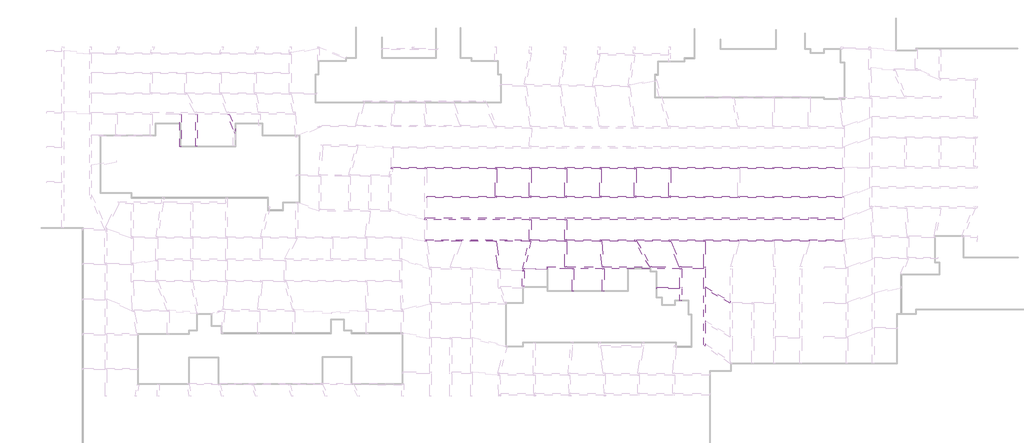
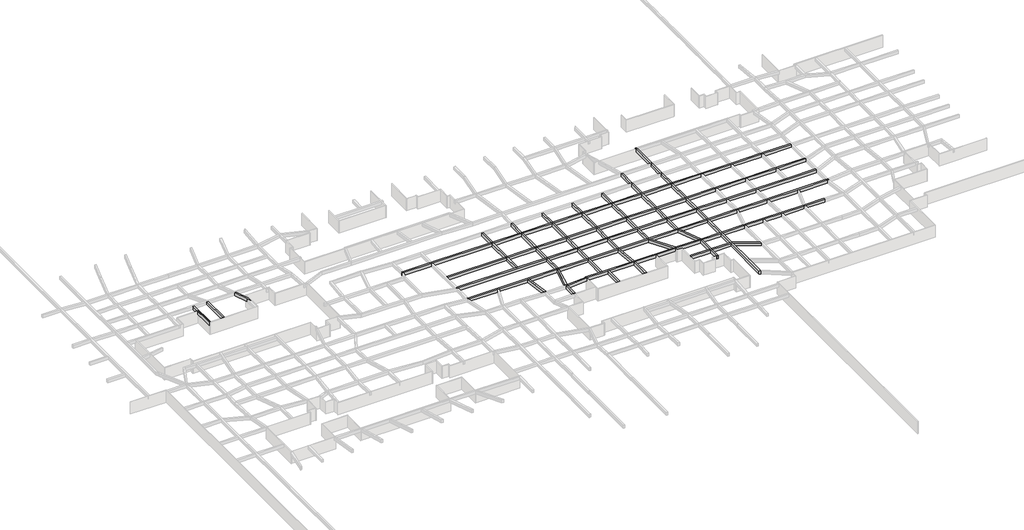
# One storey, part 18 of 45: 30 beams.
"""IFC4 building model written with IfcOpenShell, lengths in millimetres."""

from ifc_helpers import new_model, si_unit, frame, origin, place, context, project, spatial, polyline, outline, extrude, faceted_brep, element, save

model = new_model("IFC4")

# Units and contexts
model_context = context("Model", 3, world=origin())
ifc_project = project(units=[si_unit("LENGTHUNIT", "METRE", prefix="MILLI")], contexts=[model_context])

# Site, building, storey
site = spatial("IfcSite", under=ifc_project)
building = spatial("IfcBuilding", under=site)
storey = spatial("IfcBuildingStorey", under=building, Name="户型图", Elevation=0.0)

# Beams
placement = place(None, origin())
element("IfcBeam", 1, ObjectType="混凝土 - 矩形梁 : KL_beam", at=placement, inside=storey, context=model_context, shape_type="SweptSolid", body=[
    extrude(outline(polyline([(-119926.6222431, -61189.4871623), (-120326.6222431, -61189.4871623), (-120326.6222431, -53989.4871623), (-119926.6222431, -53989.4871623), (-119926.6222431, -61189.4871623)])), frame((0.0, 0.0, 2500.0), z_axis=(0.0, 0.0, 1.0), x_axis=(1.0, 0.0, 0.0)), (0.0, 0.0, 1.0), 800.0),
])
element("IfcBeam", 2, ObjectType="混凝土 - 矩形梁 : KL_beam", at=placement, inside=storey, context=model_context, shape_type="Brep", body=[
    faceted_brep([(-111449.0790859, -58416.1962178, 3300.0), (-111449.0790859, -57300.024974, 3300.0), (-112719.8754884, -53989.4871623, 3300.0), (-113148.3334859, -53989.4871623, 3300.0), (-111849.0790859, -57374.1605919, 3300.0), (-111449.0790859, -58416.1962178, 2500.0), (-113148.3334859, -53989.4871623, 2500.0), (-111849.0790859, -57374.1605919, 2500.0), (-111449.0790859, -57300.024974, 2500.0), (-112719.8754884, -53989.4871623, 2500.0)], [[[0, 1, 2, 3, 4]], [[5, 0, 4, 3, 6, 7]], [[8, 5, 7, 6, 9]], [[1, 8, 9, 2]], [[3, 2, 9, 6]], [[1, 0, 5, 8]]]),
])
element("IfcBeam", 3, ObjectType="混凝土 - 矩形梁 : KL_beam", at=placement, inside=storey, context=model_context, shape_type="SweptSolid", body=[
    extrude(outline(polyline([(-123526.6222431, -61289.4871623), (-123926.6222431, -61289.4871623), (-123926.6222431, -53989.4871623), (-123526.6222431, -53989.4871623), (-123526.6222431, -61289.4871623)])), frame((0.0, 0.0, 2500.0), z_axis=(0.0, 0.0, 1.0), x_axis=(1.0, 0.0, 0.0)), (0.0, 0.0, 1.0), 800.0),
])
element("IfcBeam", 4, ObjectType="混凝土 - 矩形梁 : KL_beam", at=placement, inside=storey, context=model_context, shape_type="Brep", body=[
    faceted_brep([(-76420.6999587, -65862.2662437, 3300.0), (-76420.6999587, -66034.5402932, 3300.0), (-76420.6999587, -66262.2662437, 3300.0), (-76069.4005138, -66262.2662437, 3300.0), (-68900.6999587, -66262.2662437, 3300.0), (-68500.6999587, -66262.2662437, 3300.0), (-53106.0296652, -66262.2662437, 3300.0), (-52706.0296652, -66262.2662437, 3300.0), (-45455.9166766, -66262.2662437, 3300.0), (-45055.9166766, -66262.2662437, 3300.0), (-37455.9166766, -66262.2662437, 3300.0), (-37055.9166766, -66262.2662437, 3300.0), (-29655.9166766, -66262.2662437, 3300.0), (-29255.9166766, -66262.2662437, 3300.0), (-21855.9166766, -66262.2662437, 3300.0), (-21455.9166766, -66262.2662437, 3300.0), (-14155.9166766, -66262.2662437, 3300.0), (-13755.9166766, -66262.2662437, 3300.0), (-6361.9880078, -66262.2662437, 3300.0), (-5961.9880078, -66262.2662437, 3300.0), (1338.0119922, -66262.2662437, 3300.0), (1738.0119922, -66262.2662437, 3300.0), (9138.0119922, -66262.2662437, 3300.0), (9538.0119922, -66262.2662437, 3300.0), (17160.5867178, -66262.2662437, 3300.0), (17560.5867178, -66262.2662437, 3300.0), (24866.4388689, -66262.2662437, 3300.0), (24866.4388689, -65862.2662437, 3300.0), (17560.5867178, -65862.2662437, 3300.0), (17160.5867178, -65862.2662437, 3300.0), (9538.0119922, -65862.2662437, 3300.0), (9138.0119922, -65862.2662437, 3300.0), (1738.0119922, -65862.2662437, 3300.0), (1338.0119922, -65862.2662437, 3300.0), (-5961.9880078, -65862.2662437, 3300.0), (-6361.9880078, -65862.2662437, 3300.0), (-13755.9166766, -65862.2662437, 3300.0), (-14155.9166766, -65862.2662437, 3300.0), (-21455.9166766, -65862.2662437, 3300.0), (-21855.9166766, -65862.2662437, 3300.0), (-29255.9166766, -65862.2662437, 3300.0), (-29655.9166766, -65862.2662437, 3300.0), (-37055.9166766, -65862.2662437, 3300.0), (-37455.9166766, -65862.2662437, 3300.0), (-45055.9166766, -65862.2662437, 3300.0), (-45455.9166766, -65862.2662437, 3300.0), (-52706.0296652, -65862.2662437, 3300.0), (-53106.0296652, -65862.2662437, 3300.0), (-68500.6999587, -65862.2662437, 3300.0), (-68900.6999587, -65862.2662437, 3300.0), (-76020.6999587, -65862.2662437, 3300.0), (-76420.6999587, -66262.2662437, 2500.0), (-76069.4005138, -66262.2662437, 2500.0), (-68900.6999587, -66262.2662437, 2500.0), (-68500.6999587, -66262.2662437, 2500.0), (-53106.0296652, -66262.2662437, 2500.0), (-52706.0296652, -66262.2662437, 2500.0), (-45455.9166766, -66262.2662437, 2500.0), (-45055.9166766, -66262.2662437, 2500.0), (-37455.9166766, -66262.2662437, 2500.0), (-37055.9166766, -66262.2662437, 2500.0), (-29655.9166766, -66262.2662437, 2500.0), (-29255.9166766, -66262.2662437, 2500.0), (-21855.9166766, -66262.2662437, 2500.0), (-21455.9166766, -66262.2662437, 2500.0), (-14155.9166766, -66262.2662437, 2500.0), (-13755.9166766, -66262.2662437, 2500.0), (-6361.9880078, -66262.2662437, 2500.0), (-5961.9880078, -66262.2662437, 2500.0), (1338.0119922, -66262.2662437, 2500.0), (1738.0119922, -66262.2662437, 2500.0), (9138.0119922, -66262.2662437, 2500.0), (9538.0119922, -66262.2662437, 2500.0), (17160.5867178, -66262.2662437, 2500.0), (17560.5867178, -66262.2662437, 2500.0), (24866.4388689, -66262.2662437, 2500.0), (-76420.6999587, -66034.5402932, 2500.0), (-76420.6999587, -65862.2662437, 2500.0), (-76020.6999587, -65862.2662437, 2500.0), (-68900.6999587, -65862.2662437, 2500.0), (-68500.6999587, -65862.2662437, 2500.0), (-53106.0296652, -65862.2662437, 2500.0), (-52706.0296652, -65862.2662437, 2500.0), (-45455.9166766, -65862.2662437, 2500.0), (-45055.9166766, -65862.2662437, 2500.0), (-37455.9166766, -65862.2662437, 2500.0), (-37055.9166766, -65862.2662437, 2500.0), (-29655.9166766, -65862.2662437, 2500.0), (-29255.9166766, -65862.2662437, 2500.0), (-21855.9166766, -65862.2662437, 2500.0), (-21455.9166766, -65862.2662437, 2500.0), (-14155.9166766, -65862.2662437, 2500.0), (-13755.9166766, -65862.2662437, 2500.0), (-6361.9880078, -65862.2662437, 2500.0), (-5961.9880078, -65862.2662437, 2500.0), (1338.0119922, -65862.2662437, 2500.0), (1738.0119922, -65862.2662437, 2500.0), (9138.0119922, -65862.2662437, 2500.0), (9538.0119922, -65862.2662437, 2500.0), (17160.5867178, -65862.2662437, 2500.0), (17560.5867178, -65862.2662437, 2500.0), (24866.4388689, -65862.2662437, 2500.0)], [[[0, 1, 2, 3, 4, 5, 6, 7, 8, 9, 10, 11, 12, 13, 14, 15, 16, 17, 18, 19, 20, 21, 22, 23, 24, 25, 26, 27, 28, 29, 30, 31, 32, 33, 34, 35, 36, 37, 38, 39, 40, 41, 42, 43, 44, 45, 46, 47, 48, 49, 50]], [[2, 51, 52, 53, 54, 55, 56, 57, 58, 59, 60, 61, 62, 63, 64, 65, 66, 67, 68, 69, 70, 71, 72, 73, 74, 75, 26, 25, 24, 23, 22, 21, 20, 19, 18, 17, 16, 15, 14, 13, 12, 11, 10, 9, 8, 7, 6, 5, 4, 3]], [[51, 76, 77, 78, 79, 80, 81, 82, 83, 84, 85, 86, 87, 88, 89, 90, 91, 92, 93, 94, 95, 96, 97, 98, 99, 100, 101, 75, 74, 73, 72, 71, 70, 69, 68, 67, 66, 65, 64, 63, 62, 61, 60, 59, 58, 57, 56, 55, 54, 53, 52]], [[77, 0, 50, 49, 48, 47, 46, 45, 44, 43, 42, 41, 40, 39, 38, 37, 36, 35, 34, 33, 32, 31, 30, 29, 28, 27, 101, 100, 99, 98, 97, 96, 95, 94, 93, 92, 91, 90, 89, 88, 87, 86, 85, 84, 83, 82, 81, 80, 79, 78]], [[2, 1, 0, 77, 76, 51]], [[27, 26, 75, 101]]]),
])
element("IfcBeam", 5, ObjectType="混凝土 - 矩形梁 : KL_beam", at=placement, inside=storey, context=model_context, shape_type="Brep", body=[
    faceted_brep([(-68500.6999587, -72411.6769994, 3300.0), (-68500.6999587, -72811.6769994, 3300.0), (-53106.0296652, -72811.6769994, 3300.0), (-52706.0296652, -72811.6769994, 3300.0), (-45455.9166766, -72811.6769994, 3300.0), (-45055.9166766, -72811.6769994, 3300.0), (-37455.9166766, -72811.6769994, 3300.0), (-37055.9166766, -72811.6769994, 3300.0), (-29655.9166766, -72811.6769994, 3300.0), (-29255.9166766, -72811.6769994, 3300.0), (-21855.9166766, -72811.6769994, 3300.0), (-21455.9166766, -72811.6769994, 3300.0), (-14155.9166766, -72811.6769994, 3300.0), (-13755.9166766, -72811.6769994, 3300.0), (-6361.9880078, -72811.6769994, 3300.0), (-5961.9880078, -72811.6769994, 3300.0), (1338.0119922, -72811.6769994, 3300.0), (1738.0119922, -72811.6769994, 3300.0), (9138.0119922, -72811.6769994, 3300.0), (9538.0119922, -72811.6769994, 3300.0), (17160.5867178, -72811.6769994, 3300.0), (17560.5867178, -72811.6769994, 3300.0), (24866.4388689, -72811.6769994, 3300.0), (24866.4388689, -72411.6769994, 3300.0), (17560.5867178, -72411.6769994, 3300.0), (17160.5867178, -72411.6769994, 3300.0), (9538.0119922, -72411.6769994, 3300.0), (9138.0119922, -72411.6769994, 3300.0), (1738.0119922, -72411.6769994, 3300.0), (1338.0119922, -72411.6769994, 3300.0), (-5961.9880078, -72411.6769994, 3300.0), (-6361.9880078, -72411.6769994, 3300.0), (-13755.9166766, -72411.6769994, 3300.0), (-14155.9166766, -72411.6769994, 3300.0), (-21455.9166766, -72411.6769994, 3300.0), (-21855.9166766, -72411.6769994, 3300.0), (-29255.9166766, -72411.6769994, 3300.0), (-29655.9166766, -72411.6769994, 3300.0), (-37055.9166766, -72411.6769994, 3300.0), (-37455.9166766, -72411.6769994, 3300.0), (-45055.9166766, -72411.6769994, 3300.0), (-45455.9166766, -72411.6769994, 3300.0), (-52706.0296652, -72411.6769994, 3300.0), (-53106.0296652, -72411.6769994, 3300.0), (-68500.6999587, -72811.6769994, 2500.0), (-53106.0296652, -72811.6769994, 2500.0), (-52706.0296652, -72811.6769994, 2500.0), (-45455.9166766, -72811.6769994, 2500.0), (-45055.9166766, -72811.6769994, 2500.0), (-37455.9166766, -72811.6769994, 2500.0), (-37055.9166766, -72811.6769994, 2500.0), (-29655.9166766, -72811.6769994, 2500.0), (-29255.9166766, -72811.6769994, 2500.0), (-21855.9166766, -72811.6769994, 2500.0), (-21455.9166766, -72811.6769994, 2500.0), (-14155.9166766, -72811.6769994, 2500.0), (-13755.9166766, -72811.6769994, 2500.0), (-6361.9880078, -72811.6769994, 2500.0), (-5961.9880078, -72811.6769994, 2500.0), (1338.0119922, -72811.6769994, 2500.0), (1738.0119922, -72811.6769994, 2500.0), (9138.0119922, -72811.6769994, 2500.0), (9538.0119922, -72811.6769994, 2500.0), (17160.5867178, -72811.6769994, 2500.0), (17560.5867178, -72811.6769994, 2500.0), (24866.4388689, -72811.6769994, 2500.0), (-68500.6999587, -72411.6769994, 2500.0), (-53106.0296652, -72411.6769994, 2500.0), (-52706.0296652, -72411.6769994, 2500.0), (-45455.9166766, -72411.6769994, 2500.0), (-45055.9166766, -72411.6769994, 2500.0), (-37455.9166766, -72411.6769994, 2500.0), (-37055.9166766, -72411.6769994, 2500.0), (-29655.9166766, -72411.6769994, 2500.0), (-29255.9166766, -72411.6769994, 2500.0), (-21855.9166766, -72411.6769994, 2500.0), (-21455.9166766, -72411.6769994, 2500.0), (-14155.9166766, -72411.6769994, 2500.0), (-13755.9166766, -72411.6769994, 2500.0), (-6361.9880078, -72411.6769994, 2500.0), (-5961.9880078, -72411.6769994, 2500.0), (1338.0119922, -72411.6769994, 2500.0), (1738.0119922, -72411.6769994, 2500.0), (9138.0119922, -72411.6769994, 2500.0), (9538.0119922, -72411.6769994, 2500.0), (17160.5867178, -72411.6769994, 2500.0), (17560.5867178, -72411.6769994, 2500.0), (24866.4388689, -72411.6769994, 2500.0)], [[[0, 1, 2, 3, 4, 5, 6, 7, 8, 9, 10, 11, 12, 13, 14, 15, 16, 17, 18, 19, 20, 21, 22, 23, 24, 25, 26, 27, 28, 29, 30, 31, 32, 33, 34, 35, 36, 37, 38, 39, 40, 41, 42, 43]], [[1, 44, 45, 46, 47, 48, 49, 50, 51, 52, 53, 54, 55, 56, 57, 58, 59, 60, 61, 62, 63, 64, 65, 22, 21, 20, 19, 18, 17, 16, 15, 14, 13, 12, 11, 10, 9, 8, 7, 6, 5, 4, 3, 2]], [[44, 66, 67, 68, 69, 70, 71, 72, 73, 74, 75, 76, 77, 78, 79, 80, 81, 82, 83, 84, 85, 86, 87, 65, 64, 63, 62, 61, 60, 59, 58, 57, 56, 55, 54, 53, 52, 51, 50, 49, 48, 47, 46, 45]], [[66, 0, 43, 42, 41, 40, 39, 38, 37, 36, 35, 34, 33, 32, 31, 30, 29, 28, 27, 26, 25, 24, 23, 87, 86, 85, 84, 83, 82, 81, 80, 79, 78, 77, 76, 75, 74, 73, 72, 71, 70, 69, 68, 67]], [[1, 0, 66, 44]], [[23, 22, 65, 87]]]),
])
element("IfcBeam", 6, ObjectType="混凝土 - 矩形梁 : KL_beam", at=placement, inside=storey, context=model_context, shape_type="Brep", body=[
    faceted_brep([(-68900.6999587, -77289.9052253, 3300.0), (-68900.6999587, -77321.0496242, 3300.0), (-68900.6999587, -77689.9052253, 3300.0), (-68500.6999587, -77689.9052253, 3300.0), (-45455.9166766, -77689.9052253, 3300.0), (-45055.9166766, -77689.9052253, 3300.0), (-37455.9166766, -77689.9052253, 3300.0), (-37055.9166766, -77689.9052253, 3300.0), (-29655.9166766, -77689.9052253, 3300.0), (-29255.9166766, -77689.9052253, 3300.0), (-21855.9166766, -77689.9052253, 3300.0), (-21455.9166766, -77689.9052253, 3300.0), (-14155.9166766, -77689.9052253, 3300.0), (-13755.9166766, -77689.9052253, 3300.0), (-6361.9880078, -77689.9052253, 3300.0), (-5961.9880078, -77689.9052253, 3300.0), (1338.0119922, -77689.9052253, 3300.0), (1738.0119922, -77689.9052253, 3300.0), (9138.0119922, -77689.9052253, 3300.0), (9538.0119922, -77689.9052253, 3300.0), (24866.4388689, -77689.9052253, 3300.0), (24866.4388689, -77289.9052253, 3300.0), (17560.5867178, -77289.9052253, 3300.0), (17160.5867178, -77289.9052253, 3300.0), (9538.0119922, -77289.9052253, 3300.0), (9138.0119922, -77289.9052253, 3300.0), (1738.0119922, -77289.9052253, 3300.0), (1338.0119922, -77289.9052253, 3300.0), (-5961.9880078, -77289.9052253, 3300.0), (-6361.9880078, -77289.9052253, 3300.0), (-13755.9166766, -77289.9052253, 3300.0), (-14155.9166766, -77289.9052253, 3300.0), (-21455.9166766, -77289.9052253, 3300.0), (-21855.9166766, -77289.9052253, 3300.0), (-29255.9166766, -77289.9052253, 3300.0), (-29655.9166766, -77289.9052253, 3300.0), (-37055.9166766, -77289.9052253, 3300.0), (-37455.9166766, -77289.9052253, 3300.0), (-45055.9166766, -77289.9052253, 3300.0), (-45455.9166766, -77289.9052253, 3300.0), (-52706.0296652, -77289.9052253, 3300.0), (-53106.0296652, -77289.9052253, 3300.0), (-68500.6999587, -77289.9052253, 3300.0), (-68900.6999587, -77689.9052253, 2500.0), (-68500.6999587, -77689.9052253, 2500.0), (-45455.9166766, -77689.9052253, 2500.0), (-45055.9166766, -77689.9052253, 2500.0), (-37455.9166766, -77689.9052253, 2500.0), (-37055.9166766, -77689.9052253, 2500.0), (-29655.9166766, -77689.9052253, 2500.0), (-29255.9166766, -77689.9052253, 2500.0), (-21855.9166766, -77689.9052253, 2500.0), (-21455.9166766, -77689.9052253, 2500.0), (-14155.9166766, -77689.9052253, 2500.0), (-13755.9166766, -77689.9052253, 2500.0), (-6361.9880078, -77689.9052253, 2500.0), (-5961.9880078, -77689.9052253, 2500.0), (1338.0119922, -77689.9052253, 2500.0), (1738.0119922, -77689.9052253, 2500.0), (9138.0119922, -77689.9052253, 2500.0), (9538.0119922, -77689.9052253, 2500.0), (24866.4388689, -77689.9052253, 2500.0), (-68900.6999587, -77321.0496242, 2500.0), (-68900.6999587, -77289.9052253, 2500.0), (-68500.6999587, -77289.9052253, 2500.0), (-53106.0296652, -77289.9052253, 2500.0), (-52706.0296652, -77289.9052253, 2500.0), (-45455.9166766, -77289.9052253, 2500.0), (-45055.9166766, -77289.9052253, 2500.0), (-37455.9166766, -77289.9052253, 2500.0), (-37055.9166766, -77289.9052253, 2500.0), (-29655.9166766, -77289.9052253, 2500.0), (-29255.9166766, -77289.9052253, 2500.0), (-21855.9166766, -77289.9052253, 2500.0), (-21455.9166766, -77289.9052253, 2500.0), (-14155.9166766, -77289.9052253, 2500.0), (-13755.9166766, -77289.9052253, 2500.0), (-6361.9880078, -77289.9052253, 2500.0), (-5961.9880078, -77289.9052253, 2500.0), (1338.0119922, -77289.9052253, 2500.0), (1738.0119922, -77289.9052253, 2500.0), (9138.0119922, -77289.9052253, 2500.0), (9538.0119922, -77289.9052253, 2500.0), (17160.5867178, -77289.9052253, 2500.0), (17560.5867178, -77289.9052253, 2500.0), (24866.4388689, -77289.9052253, 2500.0)], [[[0, 1, 2, 3, 4, 5, 6, 7, 8, 9, 10, 11, 12, 13, 14, 15, 16, 17, 18, 19, 20, 21, 22, 23, 24, 25, 26, 27, 28, 29, 30, 31, 32, 33, 34, 35, 36, 37, 38, 39, 40, 41, 42]], [[2, 43, 44, 45, 46, 47, 48, 49, 50, 51, 52, 53, 54, 55, 56, 57, 58, 59, 60, 61, 20, 19, 18, 17, 16, 15, 14, 13, 12, 11, 10, 9, 8, 7, 6, 5, 4, 3]], [[43, 62, 63, 64, 65, 66, 67, 68, 69, 70, 71, 72, 73, 74, 75, 76, 77, 78, 79, 80, 81, 82, 83, 84, 85, 61, 60, 59, 58, 57, 56, 55, 54, 53, 52, 51, 50, 49, 48, 47, 46, 45, 44]], [[63, 0, 42, 41, 40, 39, 38, 37, 36, 35, 34, 33, 32, 31, 30, 29, 28, 27, 26, 25, 24, 23, 22, 21, 85, 84, 83, 82, 81, 80, 79, 78, 77, 76, 75, 74, 73, 72, 71, 70, 69, 68, 67, 66, 65, 64]], [[2, 1, 0, 63, 62, 43]], [[21, 20, 61, 85]]]),
])
element("IfcBeam", 7, ObjectType="混凝土 - 矩形梁 : KL_beam", at=placement, inside=storey, context=model_context, shape_type="Brep", body=[
    faceted_brep([(-68721.961123, -82134.4617231, 3300.0), (-68745.1611393, -82534.4617231, 3300.0), (-68495.5196461, -82534.4617231, 3300.0), (-61086.3295601, -82534.4617231, 3300.0), (-60660.6584511, -82534.4617231, 3300.0), (-53214.7333467, -82534.4617231, 3300.0), (-52811.3449172, -82534.4617231, 3300.0), (-45507.3511364, -82534.4617231, 3300.0), (-45096.8294933, -82534.4617231, 3300.0), (-37455.9166766, -82534.4617231, 3300.0), (-37055.9166766, -82534.4617231, 3300.0), (-29638.00353, -82534.4617231, 3300.0), (-29236.2432002, -82534.4617231, 3300.0), (-21771.3867304, -82534.4617231, 3300.0), (-21309.5065151, -82534.4617231, 3300.0), (-14090.81838, -82534.4617231, 3300.0), (-13659.4044829, -82534.4617231, 3300.0), (-6361.9880078, -82534.4617231, 3300.0), (-5961.9880078, -82534.4617231, 3300.0), (1277.3669177, -82534.4617231, 3300.0), (1691.4773898, -82534.4617231, 3300.0), (9144.8742373, -82534.4617231, 3300.0), (9545.118055, -82534.4617231, 3300.0), (17090.3022302, -82534.4617231, 3300.0), (17508.5789328, -82534.4617231, 3300.0), (24889.5407453, -82534.4617231, 3300.0), (25266.4388689, -82534.4617231, 3300.0), (25266.4388689, -82511.406776, 3300.0), (25266.4388689, -82134.4617231, 3300.0), (24866.4388689, -82134.4617231, 3300.0), (9538.0119922, -82134.4617231, 3300.0), (9138.0119922, -82134.4617231, 3300.0), (1738.0119922, -82134.4617231, 3300.0), (1338.0119922, -82134.4617231, 3300.0), (-5961.9880078, -82134.4617231, 3300.0), (-6361.9880078, -82134.4617231, 3300.0), (-13755.9166766, -82134.4617231, 3300.0), (-14155.9166766, -82134.4617231, 3300.0), (-21455.9166766, -82134.4617231, 3300.0), (-21855.9166766, -82134.4617231, 3300.0), (-29255.9166766, -82134.4617231, 3300.0), (-29655.9166766, -82134.4617231, 3300.0), (-37055.9166766, -82134.4617231, 3300.0), (-37455.9166766, -82134.4617231, 3300.0), (-45055.9166766, -82134.4617231, 3300.0), (-45455.9166766, -82134.4617231, 3300.0), (-68500.6999587, -82134.4617231, 3300.0), (-68745.1611393, -82534.4617231, 2500.0), (-68495.5196461, -82534.4617231, 2500.0), (-61086.3295601, -82534.4617231, 2500.0), (-60660.6584511, -82534.4617231, 2500.0), (-53214.7333467, -82534.4617231, 2500.0), (-52811.3449172, -82534.4617231, 2500.0), (-45507.3511364, -82534.4617231, 2500.0), (-45096.8294933, -82534.4617231, 2500.0), (-37455.9166766, -82534.4617231, 2500.0), (-37055.9166766, -82534.4617231, 2500.0), (-29638.00353, -82534.4617231, 2500.0), (-29236.2432002, -82534.4617231, 2500.0), (-21771.3867304, -82534.4617231, 2500.0), (-21309.5065151, -82534.4617231, 2500.0), (-14090.81838, -82534.4617231, 2500.0), (-13659.4044829, -82534.4617231, 2500.0), (-6361.9880078, -82534.4617231, 2500.0), (-5961.9880078, -82534.4617231, 2500.0), (1277.3669177, -82534.4617231, 2500.0), (1691.4773898, -82534.4617231, 2500.0), (9144.8742373, -82534.4617231, 2500.0), (9545.118055, -82534.4617231, 2500.0), (17090.3022302, -82534.4617231, 2500.0), (17508.5789328, -82534.4617231, 2500.0), (24889.5407453, -82534.4617231, 2500.0), (25266.4388689, -82534.4617231, 2500.0), (-68721.961123, -82134.4617231, 2500.0), (-68500.6999587, -82134.4617231, 2500.0), (-45455.9166766, -82134.4617231, 2500.0), (-45055.9166766, -82134.4617231, 2500.0), (-37455.9166766, -82134.4617231, 2500.0), (-37055.9166766, -82134.4617231, 2500.0), (-29655.9166766, -82134.4617231, 2500.0), (-29255.9166766, -82134.4617231, 2500.0), (-21855.9166766, -82134.4617231, 2500.0), (-21455.9166766, -82134.4617231, 2500.0), (-14155.9166766, -82134.4617231, 2500.0), (-13755.9166766, -82134.4617231, 2500.0), (-6361.9880078, -82134.4617231, 2500.0), (-5961.9880078, -82134.4617231, 2500.0), (1338.0119922, -82134.4617231, 2500.0), (1738.0119922, -82134.4617231, 2500.0), (9138.0119922, -82134.4617231, 2500.0), (9538.0119922, -82134.4617231, 2500.0), (24866.4388689, -82134.4617231, 2500.0), (25266.4388689, -82134.4617231, 2500.0), (25266.4388689, -82511.406776, 2500.0)], [[[0, 1, 2, 3, 4, 5, 6, 7, 8, 9, 10, 11, 12, 13, 14, 15, 16, 17, 18, 19, 20, 21, 22, 23, 24, 25, 26, 27, 28, 29, 30, 31, 32, 33, 34, 35, 36, 37, 38, 39, 40, 41, 42, 43, 44, 45, 46]], [[1, 47, 48, 49, 50, 51, 52, 53, 54, 55, 56, 57, 58, 59, 60, 61, 62, 63, 64, 65, 66, 67, 68, 69, 70, 71, 72, 26, 25, 24, 23, 22, 21, 20, 19, 18, 17, 16, 15, 14, 13, 12, 11, 10, 9, 8, 7, 6, 5, 4, 3, 2]], [[47, 73, 74, 75, 76, 77, 78, 79, 80, 81, 82, 83, 84, 85, 86, 87, 88, 89, 90, 91, 92, 93, 72, 71, 70, 69, 68, 67, 66, 65, 64, 63, 62, 61, 60, 59, 58, 57, 56, 55, 54, 53, 52, 51, 50, 49, 48]], [[73, 0, 46, 45, 44, 43, 42, 41, 40, 39, 38, 37, 36, 35, 34, 33, 32, 31, 30, 29, 28, 92, 91, 90, 89, 88, 87, 86, 85, 84, 83, 82, 81, 80, 79, 78, 77, 76, 75, 74]], [[0, 73, 47, 1]], [[28, 27, 26, 72, 93, 92]]]),
])
element("IfcBeam", 8, ObjectType="混凝土 - 矩形梁 : KL_beam", at=placement, inside=storey, context=model_context, shape_type="Brep", body=[
    faceted_brep([(-41470.268972, -88390.7983183, 3300.0), (-41451.2732989, -88687.9389906, 3300.0), (-41444.7497786, -88789.9834517, 3300.0), (-41444.7497786, -88789.9834517, 2500.0), (-41451.2732989, -88687.9389906, 2500.0), (-41470.268972, -88390.7983183, 2500.0), (-41477.971202, -88391.2907081, 3300.0), (-46523.4512037, -88713.8392437, 3300.0), (-46785.1341431, -88730.5681671, 3300.0), (-46772.3615365, -89130.5681671, 3300.0), (-46578.6472042, -89118.1843555, 3300.0), (-46772.3615365, -89130.5681671, 2500.0), (-46578.6472042, -89118.1843555, 2500.0), (-46785.1341431, -88730.5681671, 2500.0), (-46523.4512037, -88713.8392437, 2500.0), (-41477.971202, -88391.2907081, 2500.0)], [[[0, 1, 2, 3, 4, 5]], [[2, 1, 0, 6, 7, 8, 9, 10]], [[3, 2, 10, 9, 11, 12]], [[5, 4, 3, 12, 11, 13, 14, 15]], [[0, 5, 15, 14, 13, 8, 7, 6]], [[8, 13, 11, 9]]]),
])
element("IfcBeam", 9, ObjectType="混凝土 - 矩形梁 : KL_beam", at=placement, inside=storey, context=model_context, shape_type="SweptSolid", body=[
    extrude(outline(polyline([(-52173.5106555, -88730.5681671), (-52408.1333935, -88718.2721105), (-53214.7333467, -82534.4617231), (-52811.3449172, -82534.4617231), (-52003.1410987, -88730.5681671), (-52173.5106555, -88730.5681671)])), frame((0.0, 0.0, 2500.0), z_axis=(0.0, 0.0, 1.0), x_axis=(1.0, 0.0, 0.0)), (0.0, 0.0, 1.0), 800.0),
])
element("IfcBeam", 10, ObjectType="混凝土 - 矩形梁 : KL_beam", at=placement, inside=storey, context=model_context, shape_type="SweptSolid", body=[
    extrude(outline(polyline([(-46578.6472042, -92630.5681671), (-46978.6472042, -92630.5681671), (-46978.6472042, -89130.5681671), (-46772.3615365, -89130.5681671), (-46578.6472042, -89118.1843555), (-46578.6472042, -92630.5681671)])), frame((0.0, 0.0, 2500.0), z_axis=(0.0, 0.0, 1.0), x_axis=(1.0, 0.0, 0.0)), (0.0, 0.0, 1.0), 800.0),
])
element("IfcBeam", 11, ObjectType="混凝土 - 矩形梁 : KL_beam", at=placement, inside=storey, context=model_context, shape_type="SweptSolid", body=[
    extrude(outline(polyline([(-46785.1341431, -88730.5681671), (-46937.8350231, -88730.5681671), (-45507.3511364, -82534.4617231), (-45096.8294933, -82534.4617231), (-46523.4512037, -88713.8392437), (-46785.1341431, -88730.5681671)])), frame((0.0, 0.0, 2500.0), z_axis=(0.0, 0.0, 1.0), x_axis=(1.0, 0.0, 0.0)), (0.0, 0.0, 1.0), 800.0),
])
element("IfcBeam", 12, ObjectType="混凝土 - 矩形梁 : KL_beam", at=placement, inside=storey, context=model_context, shape_type="SweptSolid", body=[
    extrude(outline(polyline([(-45455.9166766, -77689.9052253), (-45055.9166766, -77689.9052253), (-45055.9166766, -82134.4617231), (-45455.9166766, -82134.4617231), (-45455.9166766, -77689.9052253)])), frame((0.0, 0.0, 2500.0), z_axis=(0.0, 0.0, 1.0), x_axis=(1.0, 0.0, 0.0)), (0.0, 0.0, 1.0), 800.0),
])
element("IfcBeam", 13, ObjectType="混凝土 - 矩形梁 : KL_beam", at=placement, inside=storey, context=model_context, shape_type="SweptSolid", body=[
    extrude(outline(polyline([(-37455.9166766, -77689.9052253), (-37055.9166766, -77689.9052253), (-37055.9166766, -82134.4617231), (-37455.9166766, -82134.4617231), (-37455.9166766, -77689.9052253)])), frame((0.0, 0.0, 2500.0), z_axis=(0.0, 0.0, 1.0), x_axis=(1.0, 0.0, 0.0)), (0.0, 0.0, 1.0), 800.0),
])
element("IfcBeam", 14, ObjectType="混凝土 - 矩形梁 : KL_beam", at=placement, inside=storey, context=model_context, shape_type="SweptSolid", body=[
    extrude(outline(polyline([(-53106.0296652, -61644.2645659), (-52706.0296652, -61644.2645659), (-52706.0296652, -65862.2662437), (-53106.0296652, -65862.2662437), (-53106.0296652, -61644.2645659)])), frame((0.0, 0.0, 2500.0), z_axis=(0.0, 0.0, 1.0), x_axis=(1.0, 0.0, 0.0)), (0.0, 0.0, 1.0), 800.0),
    extrude(outline(polyline([(-52706.0296652, -77289.9052253), (-53106.0296652, -77289.9052253), (-53106.0296652, -72811.6769994), (-52706.0296652, -72811.6769994), (-52706.0296652, -77289.9052253)])), frame((0.0, 0.0, 2500.0), z_axis=(0.0, 0.0, 1.0), x_axis=(1.0, 0.0, 0.0)), (0.0, 0.0, 1.0), 800.0),
    extrude(outline(polyline([(-53106.0296652, -66262.2662437), (-52706.0296652, -66262.2662437), (-52706.0296652, -72411.6769994), (-53106.0296652, -72411.6769994), (-53106.0296652, -66262.2662437)])), frame((0.0, 0.0, 2500.0), z_axis=(0.0, 0.0, 1.0), x_axis=(1.0, 0.0, 0.0)), (0.0, 0.0, 1.0), 800.0),
])
element("IfcBeam", 15, ObjectType="混凝土 - 矩形梁 : KL_beam", at=placement, inside=storey, context=model_context, shape_type="SweptSolid", body=[
    extrude(outline(polyline([(-45455.9166766, -61644.2645659), (-45055.9166766, -61644.2645659), (-45055.9166766, -65862.2662437), (-45455.9166766, -65862.2662437), (-45455.9166766, -61644.2645659)])), frame((0.0, 0.0, 2500.0), z_axis=(0.0, 0.0, 1.0), x_axis=(1.0, 0.0, 0.0)), (0.0, 0.0, 1.0), 800.0),
    extrude(outline(polyline([(-45055.9166766, -77289.9052253), (-45455.9166766, -77289.9052253), (-45455.9166766, -72811.6769994), (-45055.9166766, -72811.6769994), (-45055.9166766, -77289.9052253)])), frame((0.0, 0.0, 2500.0), z_axis=(0.0, 0.0, 1.0), x_axis=(1.0, 0.0, 0.0)), (0.0, 0.0, 1.0), 800.0),
    extrude(outline(polyline([(-45455.9166766, -66262.2662437), (-45055.9166766, -66262.2662437), (-45055.9166766, -72411.6769994), (-45455.9166766, -72411.6769994), (-45455.9166766, -66262.2662437)])), frame((0.0, 0.0, 2500.0), z_axis=(0.0, 0.0, 1.0), x_axis=(1.0, 0.0, 0.0)), (0.0, 0.0, 1.0), 800.0),
])
element("IfcBeam", 16, ObjectType="混凝土 - 矩形梁 : KL_beam", at=placement, inside=storey, context=model_context, shape_type="SweptSolid", body=[
    extrude(outline(polyline([(-37455.9166766, -61644.2645659), (-37055.9166766, -61644.2645659), (-37055.9166766, -65862.2662437), (-37455.9166766, -65862.2662437), (-37455.9166766, -61644.2645659)])), frame((0.0, 0.0, 2500.0), z_axis=(0.0, 0.0, 1.0), x_axis=(1.0, 0.0, 0.0)), (0.0, 0.0, 1.0), 800.0),
    extrude(outline(polyline([(-37055.9166766, -77289.9052253), (-37455.9166766, -77289.9052253), (-37455.9166766, -72811.6769994), (-37055.9166766, -72811.6769994), (-37055.9166766, -77289.9052253)])), frame((0.0, 0.0, 2500.0), z_axis=(0.0, 0.0, 1.0), x_axis=(1.0, 0.0, 0.0)), (0.0, 0.0, 1.0), 800.0),
    extrude(outline(polyline([(-37455.9166766, -66262.2662437), (-37055.9166766, -66262.2662437), (-37055.9166766, -72411.6769994), (-37455.9166766, -72411.6769994), (-37455.9166766, -66262.2662437)])), frame((0.0, 0.0, 2500.0), z_axis=(0.0, 0.0, 1.0), x_axis=(1.0, 0.0, 0.0)), (0.0, 0.0, 1.0), 800.0),
])
element("IfcBeam", 17, ObjectType="混凝土 - 矩形梁 : KL_beam", at=placement, inside=storey, context=model_context, shape_type="SweptSolid", body=[
    extrude(outline(polyline([(-29655.9166766, -61644.2645659), (-29255.9166766, -61644.2645659), (-29255.9166766, -65862.2662437), (-29655.9166766, -65862.2662437), (-29655.9166766, -61644.2645659)])), frame((0.0, 0.0, 2500.0), z_axis=(0.0, 0.0, 1.0), x_axis=(1.0, 0.0, 0.0)), (0.0, 0.0, 1.0), 800.0),
    extrude(outline(polyline([(-29255.9166766, -82134.4617231), (-29655.9166766, -82134.4617231), (-29655.9166766, -77689.9052253), (-29255.9166766, -77689.9052253), (-29255.9166766, -82134.4617231)])), frame((0.0, 0.0, 2500.0), z_axis=(0.0, 0.0, 1.0), x_axis=(1.0, 0.0, 0.0)), (0.0, 0.0, 1.0), 800.0),
    extrude(outline(polyline([(-29655.9166766, -66262.2662437), (-29255.9166766, -66262.2662437), (-29255.9166766, -72411.6769994), (-29655.9166766, -72411.6769994), (-29655.9166766, -66262.2662437)])), frame((0.0, 0.0, 2500.0), z_axis=(0.0, 0.0, 1.0), x_axis=(1.0, 0.0, 0.0)), (0.0, 0.0, 1.0), 800.0),
    extrude(outline(polyline([(-29655.9166766, -72811.6769994), (-29255.9166766, -72811.6769994), (-29255.9166766, -77289.9052253), (-29655.9166766, -77289.9052253), (-29655.9166766, -72811.6769994)])), frame((0.0, 0.0, 2500.0), z_axis=(0.0, 0.0, 1.0), x_axis=(1.0, 0.0, 0.0)), (0.0, 0.0, 1.0), 800.0),
])
element("IfcBeam", 18, ObjectType="混凝土 - 矩形梁 : KL_beam", at=placement, inside=storey, context=model_context, shape_type="SweptSolid", body=[
    extrude(outline(polyline([(-21855.9166766, -61644.2645659), (-21455.9166766, -61644.2645659), (-21455.9166766, -65862.2662437), (-21855.9166766, -65862.2662437), (-21855.9166766, -61644.2645659)])), frame((0.0, 0.0, 2500.0), z_axis=(0.0, 0.0, 1.0), x_axis=(1.0, 0.0, 0.0)), (0.0, 0.0, 1.0), 800.0),
    extrude(outline(polyline([(-21455.9166766, -82134.4617231), (-21855.9166766, -82134.4617231), (-21855.9166766, -77689.9052253), (-21455.9166766, -77689.9052253), (-21455.9166766, -82134.4617231)])), frame((0.0, 0.0, 2500.0), z_axis=(0.0, 0.0, 1.0), x_axis=(1.0, 0.0, 0.0)), (0.0, 0.0, 1.0), 800.0),
    extrude(outline(polyline([(-21855.9166766, -66262.2662437), (-21455.9166766, -66262.2662437), (-21455.9166766, -72411.6769994), (-21855.9166766, -72411.6769994), (-21855.9166766, -66262.2662437)])), frame((0.0, 0.0, 2500.0), z_axis=(0.0, 0.0, 1.0), x_axis=(1.0, 0.0, 0.0)), (0.0, 0.0, 1.0), 800.0),
    extrude(outline(polyline([(-21855.9166766, -72811.6769994), (-21455.9166766, -72811.6769994), (-21455.9166766, -77289.9052253), (-21855.9166766, -77289.9052253), (-21855.9166766, -72811.6769994)])), frame((0.0, 0.0, 2500.0), z_axis=(0.0, 0.0, 1.0), x_axis=(1.0, 0.0, 0.0)), (0.0, 0.0, 1.0), 800.0),
])
element("IfcBeam", 19, ObjectType="混凝土 - 矩形梁 : KL_beam", at=placement, inside=storey, context=model_context, shape_type="SweptSolid", body=[
    extrude(outline(polyline([(-13755.9166766, -82134.4617231), (-14155.9166766, -82134.4617231), (-14155.9166766, -77689.9052253), (-13755.9166766, -77689.9052253), (-13755.9166766, -82134.4617231)])), frame((0.0, 0.0, 2500.0), z_axis=(0.0, 0.0, 1.0), x_axis=(1.0, 0.0, 0.0)), (0.0, 0.0, 1.0), 800.0),
    extrude(outline(polyline([(-14155.9166766, -57112.697306), (-13755.9166766, -57112.697306), (-13755.9166766, -61244.2645659), (-14155.9166766, -61244.2645659), (-14155.9166766, -57112.697306)])), frame((0.0, 0.0, 2500.0), z_axis=(0.0, 0.0, 1.0), x_axis=(1.0, 0.0, 0.0)), (0.0, 0.0, 1.0), 800.0),
    extrude(outline(polyline([(-14155.9166766, -61644.2645659), (-13755.9166766, -61644.2645659), (-13755.9166766, -65862.2662437), (-14155.9166766, -65862.2662437), (-14155.9166766, -61644.2645659)])), frame((0.0, 0.0, 2500.0), z_axis=(0.0, 0.0, 1.0), x_axis=(1.0, 0.0, 0.0)), (0.0, 0.0, 1.0), 800.0),
    extrude(outline(polyline([(-14155.9166766, -66262.2662437), (-13755.9166766, -66262.2662437), (-13755.9166766, -72411.6769994), (-14155.9166766, -72411.6769994), (-14155.9166766, -66262.2662437)])), frame((0.0, 0.0, 2500.0), z_axis=(0.0, 0.0, 1.0), x_axis=(1.0, 0.0, 0.0)), (0.0, 0.0, 1.0), 800.0),
    extrude(outline(polyline([(-14155.9166766, -72811.6769994), (-13755.9166766, -72811.6769994), (-13755.9166766, -77289.9052253), (-14155.9166766, -77289.9052253), (-14155.9166766, -72811.6769994)])), frame((0.0, 0.0, 2500.0), z_axis=(0.0, 0.0, 1.0), x_axis=(1.0, 0.0, 0.0)), (0.0, 0.0, 1.0), 800.0),
])
element("IfcBeam", 20, ObjectType="混凝土 - 矩形梁 : KL_beam", at=placement, inside=storey, context=model_context, shape_type="Brep", body=[
    faceted_brep([(-6361.9880078, -105772.1367475, 3300.0), (-5961.9880078, -106053.71057, 3300.0), (-5961.9880078, -105564.5441182, 3300.0), (-5961.9880078, -100834.7253412, 3300.0), (-5961.9880078, -100372.6431355, 3300.0), (-5961.9880078, -93214.7253412, 3300.0), (-5961.9880078, -92752.6431355, 3300.0), (-5961.9880078, -88687.9389906, 3300.0), (-5961.9880078, -88287.9389906, 3300.0), (-5961.9880078, -82534.4617231, 3300.0), (-6361.9880078, -82534.4617231, 3300.0), (-6361.9880078, -88287.9389906, 3300.0), (-6361.9880078, -88687.9389906, 3300.0), (-6361.9880078, -92793.9793842, 3300.0), (-6361.9880078, -93193.9793842, 3300.0), (-6361.9880078, -105772.1367475, 2500.0), (-6361.9880078, -82534.4617231, 2500.0), (-6361.9880078, -88287.9389906, 2500.0), (-6361.9880078, -88687.9389906, 2500.0), (-6361.9880078, -92793.9793842, 2500.0), (-6361.9880078, -93193.9793842, 2500.0), (-5961.9880078, -106053.71057, 2500.0), (-5961.9880078, -82534.4617231, 2500.0), (-5961.9880078, -88287.9389906, 2500.0), (-5961.9880078, -88687.9389906, 2500.0), (-5961.9880078, -92752.6431355, 2500.0), (-5961.9880078, -93214.7253412, 2500.0), (-5961.9880078, -100372.6431355, 2500.0), (-5961.9880078, -100834.7253412, 2500.0), (-5961.9880078, -105564.5441182, 2500.0)], [[[0, 1, 2, 3, 4, 5, 6, 7, 8, 9, 10, 11, 12, 13, 14]], [[15, 0, 14, 13, 12, 11, 10, 16, 17, 18, 19, 20]], [[21, 15, 20, 19, 18, 17, 16, 22, 23, 24, 25, 26, 27, 28, 29]], [[1, 21, 29, 28, 27, 26, 25, 24, 23, 22, 9, 8, 7, 6, 5, 4, 3, 2]], [[10, 9, 22, 16]], [[1, 0, 15, 21]]]),
    faceted_brep([(-6361.9880078, -57112.697306, 3300.0), (-5961.9880078, -57112.697306, 3300.0), (-5961.9880078, -57112.697306, 2500.0), (-6361.9880078, -57112.697306, 2500.0), (-5961.9880078, -61244.2645659, 3300.0), (-6361.9880078, -61244.2645659, 3300.0), (-6361.9880078, -61244.2645659, 2500.0), (-5961.9880078, -61244.2645659, 2500.0)], [[[0, 1, 2, 3]], [[4, 5, 6, 7]], [[1, 0, 5, 4]], [[0, 3, 6, 5]], [[3, 2, 7, 6]], [[2, 1, 4, 7]]]),
    faceted_brep([(-5961.9880078, -56712.697306, 3300.0), (-6361.9880078, -56712.697306, 3300.0), (-6361.9880078, -56712.697306, 2500.0), (-5961.9880078, -56712.697306, 2500.0), (-5961.9880078, -50434.4617231, 3300.0), (-5961.9880078, -50034.4617231, 3300.0), (-6361.9880078, -50034.4617231, 3300.0), (-6361.9880078, -50034.4617231, 2500.0), (-5961.9880078, -50034.4617231, 2500.0), (-5961.9880078, -50434.4617231, 2500.0)], [[[0, 1, 2, 3]], [[1, 0, 4, 5, 6]], [[2, 1, 6, 7]], [[3, 2, 7, 8, 9]], [[0, 3, 9, 8, 5, 4]], [[6, 5, 8, 7]]]),
    faceted_brep([(-6361.9880078, -61644.2645659, 3300.0), (-5961.9880078, -61644.2645659, 3300.0), (-5961.9880078, -61644.2645659, 2500.0), (-6361.9880078, -61644.2645659, 2500.0), (-5961.9880078, -65862.2662437, 3300.0), (-6361.9880078, -65862.2662437, 3300.0), (-6361.9880078, -65862.2662437, 2500.0), (-5961.9880078, -65862.2662437, 2500.0)], [[[0, 1, 2, 3]], [[4, 5, 6, 7]], [[1, 0, 5, 4]], [[0, 3, 6, 5]], [[3, 2, 7, 6]], [[2, 1, 4, 7]]]),
    faceted_brep([(-6361.9880078, -66262.2662437, 3300.0), (-5961.9880078, -66262.2662437, 3300.0), (-5961.9880078, -66262.2662437, 2500.0), (-6361.9880078, -66262.2662437, 2500.0), (-5961.9880078, -72411.6769994, 3300.0), (-6361.9880078, -72411.6769994, 3300.0), (-6361.9880078, -72411.6769994, 2500.0), (-5961.9880078, -72411.6769994, 2500.0)], [[[0, 1, 2, 3]], [[4, 5, 6, 7]], [[1, 0, 5, 4]], [[0, 3, 6, 5]], [[3, 2, 7, 6]], [[2, 1, 4, 7]]]),
    faceted_brep([(-6361.9880078, -72811.6769994, 3300.0), (-5961.9880078, -72811.6769994, 3300.0), (-5961.9880078, -72811.6769994, 2500.0), (-6361.9880078, -72811.6769994, 2500.0), (-5961.9880078, -77289.9052253, 3300.0), (-6361.9880078, -77289.9052253, 3300.0), (-6361.9880078, -77289.9052253, 2500.0), (-5961.9880078, -77289.9052253, 2500.0)], [[[0, 1, 2, 3]], [[4, 5, 6, 7]], [[1, 0, 5, 4]], [[0, 3, 6, 5]], [[3, 2, 7, 6]], [[2, 1, 4, 7]]]),
    faceted_brep([(-6361.9880078, -77689.9052253, 3300.0), (-5961.9880078, -77689.9052253, 3300.0), (-5961.9880078, -77689.9052253, 2500.0), (-6361.9880078, -77689.9052253, 2500.0), (-5961.9880078, -82134.4617231, 3300.0), (-6361.9880078, -82134.4617231, 3300.0), (-6361.9880078, -82134.4617231, 2500.0), (-5961.9880078, -82134.4617231, 2500.0)], [[[0, 1, 2, 3]], [[4, 5, 6, 7]], [[1, 0, 5, 4]], [[0, 3, 6, 5]], [[3, 2, 7, 6]], [[2, 1, 4, 7]]]),
])
element("IfcBeam", 21, ObjectType="混凝土 - 矩形梁 : KL_beam", at=placement, inside=storey, context=model_context, shape_type="Brep", body=[
    faceted_brep([(-41477.971202, -88287.9389906, 3300.0), (-41477.971202, -88287.9389906, 2500.0), (-41477.971202, -88391.2907081, 2500.0), (-41477.971202, -88391.2907081, 3300.0), (-41470.268972, -88390.7983183, 3300.0), (-41451.2732989, -88687.9389906, 3300.0), (-35863.8297061, -88687.9389906, 3300.0), (-35463.8297061, -88687.9389906, 3300.0), (-29077.9505198, -88687.9389906, 3300.0), (-28677.9505198, -88687.9389906, 3300.0), (-11669.7015983, -88687.9389906, 3300.0), (-11269.7015983, -88687.9389906, 3300.0), (-6361.9880078, -88687.9389906, 3300.0), (-6361.9880078, -88287.9389906, 3300.0), (-11334.8487771, -88287.9389906, 3300.0), (-11766.2626742, -88287.9389906, 3300.0), (-17987.7348659, -88287.9389906, 3300.0), (-18449.6150813, -88287.9389906, 3300.0), (-28695.8750901, -88287.9389906, 3300.0), (-29097.6354199, -88287.9389906, 3300.0), (-37055.9166766, -88287.9389906, 3300.0), (-37455.9166766, -88287.9389906, 3300.0), (-6361.9880078, -88287.9389906, 2500.0), (-11334.8487771, -88287.9389906, 2500.0), (-11766.2626742, -88287.9389906, 2500.0), (-17987.7348659, -88287.9389906, 2500.0), (-18449.6150813, -88287.9389906, 2500.0), (-28695.8750901, -88287.9389906, 2500.0), (-29097.6354199, -88287.9389906, 2500.0), (-37055.9166766, -88287.9389906, 2500.0), (-37455.9166766, -88287.9389906, 2500.0), (-6361.9880078, -88687.9389906, 2500.0), (-11269.7015983, -88687.9389906, 2500.0), (-11669.7015983, -88687.9389906, 2500.0), (-28677.9505198, -88687.9389906, 2500.0), (-29077.9505198, -88687.9389906, 2500.0), (-35463.8297061, -88687.9389906, 2500.0), (-35863.8297061, -88687.9389906, 2500.0), (-41451.2732989, -88687.9389906, 2500.0), (-41470.268972, -88390.7983183, 2500.0)], [[[0, 1, 2, 3]], [[0, 3, 4, 5, 6, 7, 8, 9, 10, 11, 12, 13, 14, 15, 16, 17, 18, 19, 20, 21]], [[1, 0, 21, 20, 19, 18, 17, 16, 15, 14, 13, 22, 23, 24, 25, 26, 27, 28, 29, 30]], [[2, 1, 30, 29, 28, 27, 26, 25, 24, 23, 22, 31, 32, 33, 34, 35, 36, 37, 38, 39]], [[5, 38, 37, 36, 35, 34, 33, 32, 31, 12, 11, 10, 9, 8, 7, 6]], [[4, 39, 38, 5]], [[39, 4, 3, 2]], [[13, 12, 31, 22]]]),
    faceted_brep([(20722.028798, -88687.9389906, 3300.0), (20722.028798, -88687.9389906, 2500.0), (20722.028798, -88287.9389906, 2500.0), (20722.028798, -88287.9389906, 3300.0), (-5961.9880078, -88687.9389906, 3300.0), (-5961.9880078, -88287.9389906, 3300.0), (-5961.9880078, -88287.9389906, 2500.0), (-5961.9880078, -88687.9389906, 2500.0), (15749.5644071, -88287.9389906, 3300.0), (15331.2877045, -88287.9389906, 3300.0), (9746.0339084, -88287.9389906, 3300.0), (9345.7900907, -88287.9389906, 3300.0), (149.8378023, -88287.9389906, 3300.0), (-264.2726698, -88287.9389906, 3300.0), (-310.8072722, -88687.9389906, 3300.0), (89.1927278, -88687.9389906, 3300.0), (4489.1927278, -88687.9389906, 3300.0), (4889.1927278, -88687.9389906, 3300.0), (9352.8961535, -88687.9389906, 3300.0), (9752.8961535, -88687.9389906, 3300.0), (15279.3735446, -88687.9389906, 3300.0), (15679.3735446, -88687.9389906, 3300.0), (15749.5644071, -88287.9389906, 2500.0), (15331.2877045, -88287.9389906, 2500.0), (9746.0339084, -88287.9389906, 2500.0), (9345.7900907, -88287.9389906, 2500.0), (149.8378023, -88287.9389906, 2500.0), (-264.2726698, -88287.9389906, 2500.0), (15679.3735446, -88687.9389906, 2500.0), (15279.3735446, -88687.9389906, 2500.0), (9752.8961535, -88687.9389906, 2500.0), (9352.8961535, -88687.9389906, 2500.0), (4889.1927278, -88687.9389906, 2500.0), (4489.1927278, -88687.9389906, 2500.0), (89.1927278, -88687.9389906, 2500.0), (-310.8072722, -88687.9389906, 2500.0)], [[[0, 1, 2, 3]], [[4, 5, 6, 7]], [[0, 3, 8, 9, 10, 11, 12, 13, 5, 4, 14, 15, 16, 17, 18, 19, 20, 21]], [[3, 2, 22, 23, 24, 25, 26, 27, 6, 5, 13, 12, 11, 10, 9, 8]], [[2, 1, 28, 29, 30, 31, 32, 33, 34, 35, 7, 6, 27, 26, 25, 24, 23, 22]], [[1, 0, 21, 20, 19, 18, 17, 16, 15, 14, 4, 7, 35, 34, 33, 32, 31, 30, 29, 28]]]),
])
element("IfcBeam", 22, ObjectType="混凝土 - 矩形梁 : KL_beam", at=placement, inside=storey, context=model_context, shape_type="SweptSolid", body=[
    extrude(outline(polyline([(-29638.00353, -82534.4617231), (-29236.2432002, -82534.4617231), (-28695.8750901, -88287.9389906), (-29097.6354199, -88287.9389906), (-29638.00353, -82534.4617231)])), frame((0.0, 0.0, 2500.0), z_axis=(0.0, 0.0, 1.0), x_axis=(1.0, 0.0, 0.0)), (0.0, 0.0, 1.0), 800.0),
])
element("IfcBeam", 23, ObjectType="混凝土 - 矩形梁 : KL_beam", at=placement, inside=storey, context=model_context, shape_type="SweptSolid", body=[
    extrude(outline(polyline([(-21771.3867304, -82534.4617231), (-21309.5065151, -82534.4617231), (-17987.7348659, -88287.9389906), (-18449.6150813, -88287.9389906), (-21771.3867304, -82534.4617231)])), frame((0.0, 0.0, 2500.0), z_axis=(0.0, 0.0, 1.0), x_axis=(1.0, 0.0, 0.0)), (0.0, 0.0, 1.0), 800.0),
])
element("IfcBeam", 24, ObjectType="混凝土 - 矩形梁 : KL_beam", at=placement, inside=storey, context=model_context, shape_type="SweptSolid", body=[
    extrude(outline(polyline([(-14090.81838, -82534.4617231), (-13659.4044829, -82534.4617231), (-11334.8487771, -88287.9389906), (-11766.2626742, -88287.9389906), (-14090.81838, -82534.4617231)])), frame((0.0, 0.0, 2500.0), z_axis=(0.0, 0.0, 1.0), x_axis=(1.0, 0.0, 0.0)), (0.0, 0.0, 1.0), 800.0),
])
element("IfcBeam", 25, ObjectType="混凝土 - 矩形梁 : KL_beam", at=placement, inside=storey, context=model_context, shape_type="SweptSolid", body=[
    extrude(outline(polyline([(-5961.9880078, -93214.7253412), (-5961.9880078, -92752.6431355), (-310.8072722, -96021.0575371), (-310.8072722, -96483.1397428), (-5961.9880078, -93214.7253412)])), frame((0.0, 0.0, 2500.0), z_axis=(0.0, 0.0, 1.0), x_axis=(1.0, 0.0, 0.0)), (0.0, 0.0, 1.0), 800.0),
])
element("IfcBeam", 26, ObjectType="混凝土 - 矩形梁 : KL_beam", at=placement, inside=storey, context=model_context, shape_type="Brep", body=[
    faceted_brep([(-11269.7015983, -95887.9994844, 3300.0), (-11669.7015983, -95887.9994844, 3300.0), (-11669.7015983, -95887.9994844, 2500.0), (-11269.7015983, -95887.9994844, 2500.0), (-11269.7015983, -93193.9793842, 3300.0), (-11269.7015983, -92793.9793842, 3300.0), (-11269.7015983, -88687.9389906, 3300.0), (-11669.7015983, -88687.9389906, 3300.0), (-11669.7015983, -92793.9793842, 3300.0), (-11669.7015983, -93193.9793842, 3300.0), (-11669.7015983, -88687.9389906, 2500.0), (-11669.7015983, -92793.9793842, 2500.0), (-11669.7015983, -93193.9793842, 2500.0), (-11269.7015983, -88687.9389906, 2500.0), (-11269.7015983, -92793.9793842, 2500.0), (-11269.7015983, -93193.9793842, 2500.0)], [[[0, 1, 2, 3]], [[1, 0, 4, 5, 6, 7, 8, 9]], [[2, 1, 9, 8, 7, 10, 11, 12]], [[3, 2, 12, 11, 10, 13, 14, 15]], [[0, 3, 15, 14, 13, 6, 5, 4]], [[7, 6, 13, 10]]]),
])
element("IfcBeam", 27, ObjectType="混凝土 - 矩形梁 : KL_beam", at=placement, inside=storey, context=model_context, shape_type="SweptSolid", body=[
    extrude(outline(polyline([(-16840.0302297, -93193.9793842), (-16840.0302297, -92793.9793842), (-11669.7015983, -92793.9793842), (-11669.7015983, -93193.9793842), (-16840.0302297, -93193.9793842)])), frame((0.0, 0.0, 2500.0), z_axis=(0.0, 0.0, 1.0), x_axis=(1.0, 0.0, 0.0)), (0.0, 0.0, 1.0), 800.0),
    extrude(outline(polyline([(-6361.9880078, -92793.9793842), (-6361.9880078, -93193.9793842), (-11269.7015983, -93193.9793842), (-11269.7015983, -92793.9793842), (-6361.9880078, -92793.9793842)])), frame((0.0, 0.0, 2500.0), z_axis=(0.0, 0.0, 1.0), x_axis=(1.0, 0.0, 0.0)), (0.0, 0.0, 1.0), 800.0),
])
element("IfcBeam", 28, ObjectType="混凝土 - 矩形梁 : KL_beam", at=placement, inside=storey, context=model_context, shape_type="SweptSolid", body=[
    extrude(outline(polyline([(-28677.9505198, -93688.0490958), (-29077.9505198, -93688.0490958), (-29077.9505198, -88687.9389906), (-28677.9505198, -88687.9389906), (-28677.9505198, -93688.0490958)])), frame((0.0, 0.0, 2500.0), z_axis=(0.0, 0.0, 1.0), x_axis=(1.0, 0.0, 0.0)), (0.0, 0.0, 1.0), 800.0),
])
element("IfcBeam", 29, ObjectType="混凝土 - 矩形梁 : KL_beam", at=placement, inside=storey, context=model_context, shape_type="SweptSolid", body=[
    extrude(outline(polyline([(-35463.8297061, -93682.1348661), (-35863.8297061, -93682.1348661), (-35863.8297061, -88687.9389906), (-35463.8297061, -88687.9389906), (-35463.8297061, -93682.1348661)])), frame((0.0, 0.0, 2500.0), z_axis=(0.0, 0.0, 1.0), x_axis=(1.0, 0.0, 0.0)), (0.0, 0.0, 1.0), 800.0),
])
element("IfcBeam", 30, ObjectType="混凝土 - 矩形梁 : KL_beam", at=placement, inside=storey, context=model_context, shape_type="SweptSolid", body=[
    extrude(outline(polyline([(-37455.9166766, -82534.4617231), (-37055.9166766, -82534.4617231), (-37055.9166766, -88287.9389906), (-37455.9166766, -88287.9389906), (-37455.9166766, -82534.4617231)])), frame((0.0, 0.0, 2500.0), z_axis=(0.0, 0.0, 1.0), x_axis=(1.0, 0.0, 0.0)), (0.0, 0.0, 1.0), 800.0),
])

save(model, "model.ifc")

# Revit data of these elements
# Type "混凝土 - 矩形梁 : KL_beam"
#   Length [instance default] = 1524 mm
#   b = 400 mm
#   h = 800 mm
#   Structural Material [instance default] = 混凝土 - 现场浇注混凝土
#   Assembly Code = ""
# Elements 1, 2, 3, 4, 5, 6, 7, 8, 9, 10, 11, 12, 13, 14, 15, 16, 17, 18, 19, 20, 21, 22, 23, 24, 25, 26, 27, 28, 29, 30 (IfcBeam, "混凝土 - 矩形梁 : KL_beam")
#   Comments = ""
#   Structural Material = none
#   Phase Created = 新构造
# Materials
#   "混凝土 - 现场浇注混凝土": class "混凝土", colour RGB 192 192 192, transparency 0
